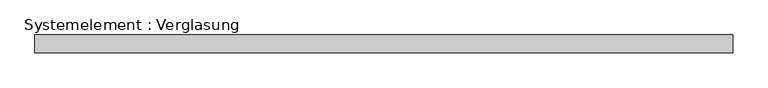
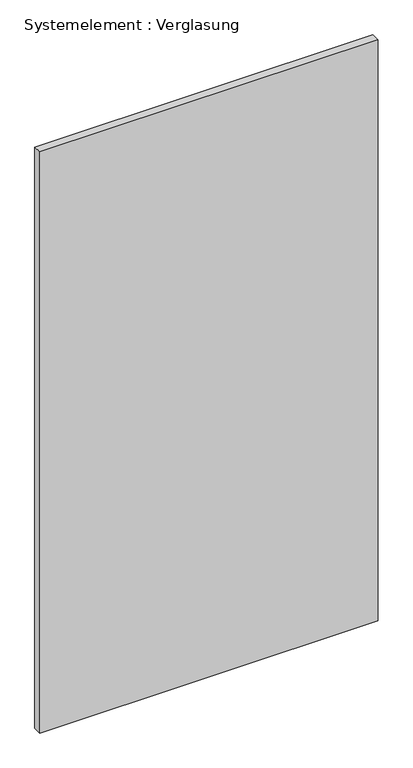
"""IFC4 building model written with IfcOpenShell, lengths in millimetres: plate geometry, Systemelement : Verglasung."""

from ifc_helpers import new_model, si_unit, origin, origin_with_axes, place, context, project, spatial, polyline, outline, extrude, source, transform, mapped, element, save


def systemelement_verglasung_d38c8d2b(model_context):
    return source(origin(), model_context, "Body", "SweptSolid", [
        extrude(outline(polyline([(595.0, -15.0), (-595.0, -15.0), (-595.0, 15.0), (595.0, 15.0), (595.0, -15.0)])), origin_with_axes(), (0.0, 0.0, 1.0), 2160.0),
    ])


if __name__ == "__main__":
    model = new_model("IFC4")
    model_context = context("Model", 3, world=origin())
    ifc_project = project(units=[si_unit("LENGTHUNIT", "METRE", prefix="MILLI")], contexts=[model_context])
    site = spatial("IfcSite", under=ifc_project)
    building = spatial("IfcBuilding", under=site)
    placement = place(None, origin())
    systemelement_verglasung_shape = systemelement_verglasung_d38c8d2b(model_context)
    element("IfcPlate", 1, ObjectType="Systemelement : Verglasung", at=placement, inside=building, context=model_context, shape_type="MappedRepresentation", body=[
        mapped(systemelement_verglasung_shape, transform((0.0, 0.0, 0.0), x_axis=(1.0, 0.0, 0.0), y_axis=(0.0, 1.0, 0.0), z_axis=(0.0, 0.0, 1.0))),
    ])
    save(model, "model.ifc")

# Revit data of these elements
# Type "Systemelement : Verglasung"
#   Construction Type Id = "GSP4R"
#   Analytic Construction = "1/8 Zoll Pilkington-Verglasung einfach"
#   Visual Light Transmittance = 0.9
#   Solar Heat Gain Coefficient = 0.86
#   Heat Transfer Coefficient (U) = 6.7069 W/(m²·K)
# Element 1 (IfcPlate, "Systemelement : Verglasung")
#   Materials on its faces: "Glas"
# Materials
#   "Glas": class "Glas", colour RGB 0 0 255, transparency 0.75, Comments = "Render-Darstellung nicht aktualisiert ", Cost = 0
